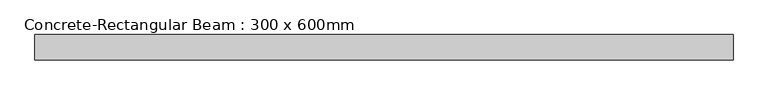
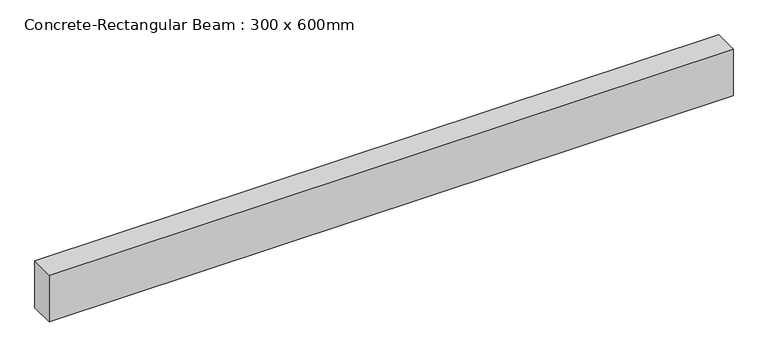
"""IFC4 building model written with IfcOpenShell, lengths in millimetres: beam geometry, Concrete-Rectangular Beam : 300 x 600mm."""

import ifcopenshell
import ifcopenshell.guid

model = None  # the IFC model being written
_history = None  # IfcOwnerHistory: only IFC2X3 demands one
_inside = {}  # id of a spatial element -> (the spatial element, [elements in it])
_under = {}  # id of a project, library or spatial element -> (it, [spatial elements below it])
_declared = {}  # id of a project -> (the project, [libraries it declares])
_typed = {}  # id of a type object -> (the type object, [elements of that type])
_made_of = {}  # id of a material, layer set ... -> (it, [elements and type objects made of it])


def new_model(schema):
    """Start an empty IFC model of exactly this schema.

    Asked for "IFC4X3", IfcOpenShell would pick the latest addendum, in which some entities
    have other attributes; the version numbers below select the first issue.
    IFC2X3 requires an IfcOwnerHistory on every rooted entity: one is made here for all.
    """
    global model, _history
    if schema == "IFC4X3":
        model = ifcopenshell.file(schema_version=(4, 3, 0, 0))
    else:
        model = ifcopenshell.file(schema=schema)
    _inside.clear()
    _under.clear()
    _declared.clear()
    _typed.clear()
    _made_of.clear()
    _history = None
    if model.schema == "IFC2X3":
        org = make("IfcOrganization", Name="unknown")
        user = make(
            "IfcPersonAndOrganization",
            ThePerson=make("IfcPerson", FamilyName="unknown"),
            TheOrganization=org,
        )
        app = make(
            "IfcApplication",
            ApplicationDeveloper=org,
            Version="unknown",
            ApplicationFullName="unknown",
            ApplicationIdentifier="unknown",
        )
        _history = make(
            "IfcOwnerHistory",
            OwningUser=user,
            OwningApplication=app,
            ChangeAction="ADDED",
            CreationDate=0,
        )
    return model


def make(cls, **values):
    """One entity of the class cls with the attributes given. An attribute that is None is left unset."""
    return model.create_entity(
        cls, **{name: value for name, value in values.items() if value is not None}
    )


def rooted(cls, **values):
    """An entity with a GlobalId (a new one), such as an element, a storey or a relation."""
    return make(cls, GlobalId=ifcopenshell.guid.new(), OwnerHistory=_history, **values)


def si_unit(unit_type, name, prefix=None):
    """IfcSIUnit, for example si_unit("LENGTHUNIT", "METRE", prefix="MILLI")."""
    return make("IfcSIUnit", UnitType=unit_type, Prefix=prefix, Name=name)


def assignment(units):
    """IfcUnitAssignment: the units of a project."""
    return None if units is None else make("IfcUnitAssignment", Units=units)


def point(xyz):
    """IfcCartesianPoint."""
    return None if xyz is None else make("IfcCartesianPoint", Coordinates=xyz)


def direction(xyz):
    """IfcDirection."""
    return None if xyz is None else make("IfcDirection", DirectionRatios=xyz)


def frame(location, z_axis=None, x_axis=None):
    """IfcAxis2Placement3D, a coordinate frame: its origin and axes. An axis left out is left unset."""
    return make(
        "IfcAxis2Placement3D",
        Location=point(location),
        Axis=direction(z_axis),
        RefDirection=direction(x_axis),
    )


def origin():
    """The frame at (0, 0, 0) with its axes left unset."""
    return frame((0.0, 0.0, 0.0))


def place(relative_to, where):
    """IfcLocalPlacement: puts the frame where relative to a parent placement (None: the world)."""
    return make(
        "IfcLocalPlacement", PlacementRelTo=relative_to, RelativePlacement=where
    )


def context(
    kind, dimensions, precision=None, world=None, true_north=None, identifier=None
):
    """IfcGeometricRepresentationContext, for example the 3D "Model" context."""
    return make(
        "IfcGeometricRepresentationContext",
        ContextIdentifier=identifier,
        ContextType=kind,
        CoordinateSpaceDimension=dimensions,
        Precision=precision,
        WorldCoordinateSystem=world,
        TrueNorth=true_north,
    )


def project(units=None, contexts=None):
    """IfcProject with its units and contexts."""
    return rooted(
        "IfcProject",
        Name="project",
        RepresentationContexts=contexts,
        UnitsInContext=assignment(units),
    )


def spatial(cls, under=None, at=None, **own):
    """A site, building, storey or space (cls), placed at a placement, below another one or the project."""
    s = rooted(cls, ObjectPlacement=at, **own)
    if under is not None:
        _under.setdefault(under.id(), (under, []))[1].append(s)
    return s


def polyline(points):
    """IfcPolyline through the points."""
    return make("IfcPolyline", Points=[point(p) for p in points])


def outline(outer, holes=None, kind="AREA"):
    """IfcArbitraryClosedProfileDef: a profile drawn as a closed curve; with holes, ...WithVoids."""
    if holes is None:
        return make("IfcArbitraryClosedProfileDef", ProfileType=kind, OuterCurve=outer)
    return make(
        "IfcArbitraryProfileDefWithVoids",
        ProfileType=kind,
        OuterCurve=outer,
        InnerCurves=holes,
    )


def extrude(swept, where, along, depth):
    """IfcExtrudedAreaSolid: the profile swept, set in the frame where, extruded along a direction by depth."""
    return make(
        "IfcExtrudedAreaSolid",
        SweptArea=swept,
        Position=where,
        ExtrudedDirection=direction(along),
        Depth=depth,
    )


def shape(context_of_items, identifier, shape_type, items):
    """IfcShapeRepresentation: the items that make up one representation, for example the "Body"."""
    return make(
        "IfcShapeRepresentation",
        ContextOfItems=context_of_items,
        RepresentationIdentifier=identifier,
        RepresentationType=shape_type,
        Items=items,
    )


def source(mapping_origin, context_of_items, identifier, shape_type, items):
    """IfcRepresentationMap: a shape defined once, which mapped items show again and again."""
    return make(
        "IfcRepresentationMap",
        MappingOrigin=mapping_origin,
        MappedRepresentation=shape(context_of_items, identifier, shape_type, items),
    )


def transform(
    local_origin,
    x_axis=None,
    y_axis=None,
    z_axis=None,
    scale=None,
    scale2=None,
    scale3=None,
    uniform=True,
):
    """IfcCartesianTransformationOperator3D, or its non-uniform kind. x_axis, y_axis, z_axis: its Axis1, 2, 3."""
    if uniform:
        return make(
            "IfcCartesianTransformationOperator3D",
            Axis1=direction(x_axis),
            Axis2=direction(y_axis),
            LocalOrigin=point(local_origin),
            Scale=scale,
            Axis3=direction(z_axis),
        )
    return make(
        "IfcCartesianTransformationOperator3DnonUniform",
        Axis1=direction(x_axis),
        Axis2=direction(y_axis),
        LocalOrigin=point(local_origin),
        Scale=scale,
        Axis3=direction(z_axis),
        Scale2=scale2,
        Scale3=scale3,
    )


def mapped(mapping_source, mapping_target):
    """IfcMappedItem: shows the shape of a source again, moved by a transform."""
    return make(
        "IfcMappedItem", MappingSource=mapping_source, MappingTarget=mapping_target
    )


def made_of(thing, what):
    """Note that an element or type object is made of a material, layer set ...; save() writes the relation."""
    if what is not None:
        _made_of.setdefault(what.id(), (what, []))[1].append(thing)
    return thing


def element(
    cls,
    number,
    at=None,
    inside=None,
    cuts=None,
    type_object=None,
    material=None,
    context=None,
    identifier="Body",
    shape_type=None,
    held_by="IfcProductDefinitionShape",
    body=None,
    shapes=None,
    **own,
):
    """One element of the class cls, such as IfcWall. Its Tag is "e" and its number.

    at: its placement. inside: the storey or other place that contains it. cuts: it is an
    opening in that element (IfcRelVoidsElement). A single representation is given by context,
    identifier, shape_type and body (its items); several are given by shapes. held_by: the class
    of the entity that holds the representations. save() writes the other relations.
    """
    e = rooted(cls, Tag="e%d" % number, ObjectPlacement=at, **own)
    if body is not None:
        shapes = [shape(context, identifier, shape_type, body)]
    if shapes is not None:
        e.Representation = make(held_by, Representations=shapes)
    if inside is not None:
        _inside.setdefault(inside.id(), (inside, []))[1].append(e)
    if cuts is not None:
        rooted(
            "IfcRelVoidsElement", RelatingBuildingElement=cuts, RelatedOpeningElement=e
        )
    if type_object is not None:
        _typed.setdefault(type_object.id(), (type_object, []))[1].append(e)
    return made_of(e, material)


def aggregate(whole, parts):
    """IfcRelAggregates: a whole, such as a stair, and the parts it consists of."""
    return rooted("IfcRelAggregates", RelatingObject=whole, RelatedObjects=parts)


def save(model, path):
    """Write the relations noted so far, then the file.

    IfcRelAggregates (storeys below a building ...), IfcRelContainedInSpatialStructure (elements
    in a storey), IfcRelDefinesByType, IfcRelAssociatesMaterial and IfcRelDeclares: one each for
    every whole, place, type object, material and project.
    """
    for whole, parts in _under.values():
        aggregate(whole, parts)
    for where, things in _inside.values():
        rooted(
            "IfcRelContainedInSpatialStructure",
            RelatedElements=things,
            RelatingStructure=where,
        )
    for kind, things in _typed.values():
        rooted("IfcRelDefinesByType", RelatedObjects=things, RelatingType=kind)
    for what, things in _made_of.values():
        rooted("IfcRelAssociatesMaterial", RelatedObjects=things, RelatingMaterial=what)
    for by, libraries in _declared.values():
        rooted("IfcRelDeclares", RelatingContext=by, RelatedDefinitions=libraries)
    model.write(path)


def concrete_rectangular_beam_300_x_600mm_b1d28744(model_context):
    return source(origin(), model_context, "Body", "SweptSolid", [
        extrude(outline(polyline([(4150.0, 150.0), (4150.0, -150.0), (-4150.0, -150.0), (-4150.0, 150.0), (4150.0, 150.0)])), frame((0.0, 0.0, -300.0), z_axis=(0.0, 0.0, 1.0), x_axis=(1.0, 0.0, 0.0)), (0.0, 0.0, 1.0), 600.0),
    ])


if __name__ == "__main__":
    model = new_model("IFC4")
    model_context = context("Model", 3, world=origin())
    ifc_project = project(units=[si_unit("LENGTHUNIT", "METRE", prefix="MILLI")], contexts=[model_context])
    site = spatial("IfcSite", under=ifc_project)
    building = spatial("IfcBuilding", under=site)
    placement = place(None, origin())
    concrete_rectangular_beam_300_x_600mm_shape = concrete_rectangular_beam_300_x_600mm_b1d28744(model_context)
    element("IfcBeam", 1, ObjectType="Concrete-Rectangular Beam : 300 x 600mm", at=placement, inside=building, context=model_context, shape_type="MappedRepresentation", body=[
        mapped(concrete_rectangular_beam_300_x_600mm_shape, transform((0.0, 0.0, 0.0), x_axis=(1.0, 0.0, 0.0), y_axis=(0.0, 1.0, 0.0), z_axis=(0.0, 0.0, 1.0))),
    ])
    save(model, "model.ifc")

# Revit data of these elements
# Type "Concrete-Rectangular Beam : 300 x 600mm"
#   Length [instance default] = 1524 mm
#   b = 300 mm
#   h = 600 mm
#   Structural Material [instance default] = Concrete, Cast-in-Place gray
#   Assembly Code = ""
# Element 1 (IfcBeam, "Concrete-Rectangular Beam : 300 x 600mm")
#   Materials on its faces: "Concrete, Cast-in-Place gray"
# Materials
#   "Concrete, Cast-in-Place gray": class "Concrete", colour RGB 192 192 192, transparency 0, Description = "Cast-in-place concrete", Cost = 0
